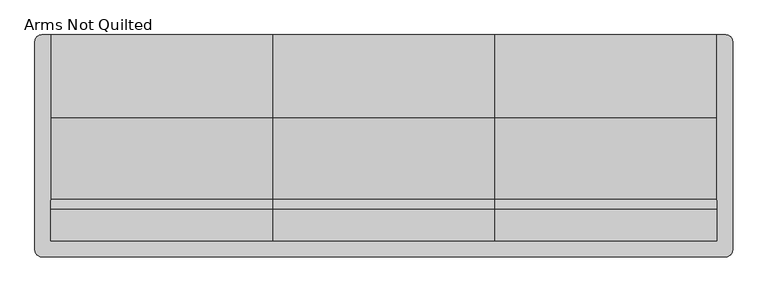
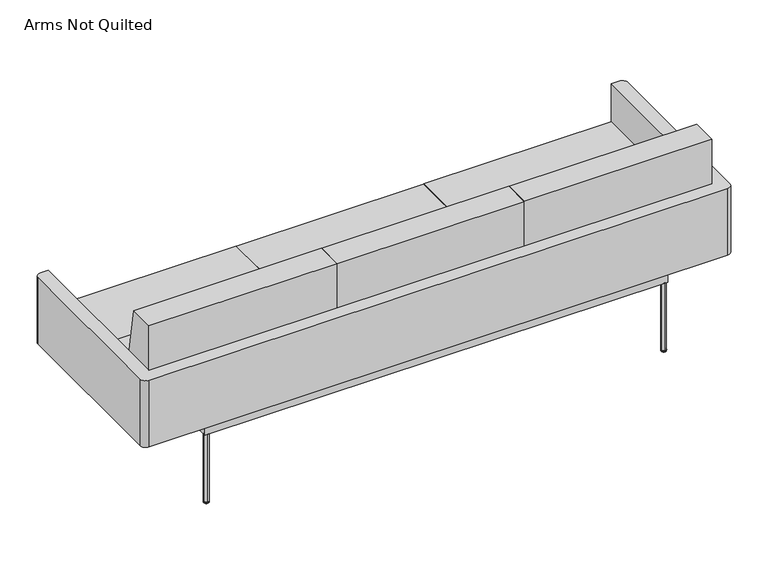
"""IFC4 building model written with IfcOpenShell, lengths in millimetres: furniture geometry, HermanMiller_Collection_Tuxedo_Sofa : Arms Not Quilted."""

from ifc_helpers import new_model, si_unit, point, frame, frame_2d, origin, place, context, project, spatial, polyline, circle_curve, ellipse_curve, trimmed, segment, composite_curve, outline, extrude, source, transform, mapped, element, save
from ifc_brep_helpers import plane_surface, revolved_surface, advanced_brep


def arms_not_quilted_b01c5f5b(model_context):
    return source(origin(), model_context, "Body", "SolidModel", [
        extrude(outline(polyline([(-172.790312, 570.0407405), (-172.790312, 357.1875), (-305.047338, 357.1875), (-305.047338, 761.9999879), (-204.8303749, 761.9999879), (-172.790312, 570.0407405)])), frame((355.8486449, 0.0, 0.0), z_axis=(1.0, 0.0, 0.0), x_axis=(0.0, 1.0, 0.0)), (0.0, 0.0, 1.0), 711.3174324),
        extrude(outline(polyline([(-204.8303749, 761.9999879), (-172.790312, 570.0407405), (-172.790312, 357.1875), (-305.047338, 357.1875), (-305.047338, 761.9999879), (-204.8303749, 761.9999879)])), frame((-1067.1660773, 0.0, 0.0), z_axis=(1.0, 0.0, 0.0), x_axis=(0.0, 1.0, 0.0)), (0.0, 0.0, 1.0), 711.3174324),
        extrude(outline(polyline([(-172.790312, 570.0407405), (-172.790312, 357.1875), (-305.047338, 357.1875), (-305.047338, 761.9999879), (-204.8303749, 761.9999879), (-172.790312, 570.0407405)])), frame((-354.5786449, 0.0, 0.0), z_axis=(1.0, 0.0, 0.0), x_axis=(0.0, 1.0, 0.0)), (0.0, 0.0, 1.0), 709.1572898),
        extrude(outline(polyline([(355.847338, 357.1875), (-172.790312, 357.1875), (-172.790312, 408.4192229), (89.4717005, 431.3641497), (355.847338, 431.3641497), (355.847338, 357.1875)])), frame((355.8486449, 0.0, 0.0), z_axis=(1.0, 0.0, 0.0), x_axis=(0.0, 1.0, 0.0)), (0.0, 0.0, 1.0), 711.3174324),
        extrude(outline(polyline([(355.847338, 431.3641497), (355.847338, 357.1875), (-172.790312, 357.1875), (-172.790312, 408.4192229), (89.4717005, 431.3641497), (355.847338, 431.3641497)])), frame((-1067.1660773, 0.0, 0.0), z_axis=(1.0, 0.0, 0.0), x_axis=(0.0, 1.0, 0.0)), (0.0, 0.0, 1.0), 711.3174324),
        extrude(outline(polyline([(355.847338, 357.1875), (-172.790312, 357.1875), (-172.790312, 408.4192229), (89.4717005, 431.3641497), (355.847338, 431.3641497), (355.847338, 357.1875)])), frame((-354.5786449, 0.0, 0.0), z_axis=(1.0, 0.0, 0.0), x_axis=(0.0, 1.0, 0.0)), (0.0, 0.0, 1.0), 709.1572898),
        advanced_brep(
        [(-862.2241883, 239.6951247, 0.0), (-866.0073712, 239.6951247, 0.0), (-869.7905542, 239.6951247, 0.0), (-856.4823712, 239.6951247, 3.1750001), (-875.5323712, 239.6951247, 3.1750001), (-856.351925, 239.6951247, 6.4931848), (-875.6628174, 239.6951247, 6.4931848), (-861.8574966, 239.6951247, 9.5049435), (-870.1572459, 239.6951247, 9.5049435), (-866.0073712, 239.6951247, 9.5049435)],
        [
            (0, 1),
            (1, 2),
            (2, 0, circle_curve(frame((-866.0073712, 239.6951247, 0.0), z_axis=(0.0, 0.0, -1.0), x_axis=(-1.0, 0.0, 0.0)), 3.783183)),
            (0, 2, circle_curve(frame((-866.0073712, 239.6951247, 0.0), z_axis=(0.0, 0.0, -1.0), x_axis=(-1.0, 0.0, 0.0)), 3.783183)),
            (3, 0, circle_curve(frame((-862.2241883, 239.6951247, 6.7793838), z_axis=(0.0, 1.0, 0.0), x_axis=(1.0, 0.0, 0.0)), 6.7793838)),
            (2, 4, circle_curve(frame((-869.7905542, 239.6951247, 6.7793838), z_axis=(0.0, 1.0, 0.0), x_axis=(-1.0, 0.0, 0.0)), 6.7793838)),
            (4, 3, circle_curve(frame((-866.0073712, 239.6951247, 3.1750001), z_axis=(0.0, 0.0, -1.0), x_axis=(-1.0, 0.0, 0.0)), 9.525)),
            (3, 4, circle_curve(frame((-866.0073712, 239.6951247, 3.1750001), z_axis=(0.0, 0.0, -1.0), x_axis=(-1.0, 0.0, 0.0)), 9.525)),
            (5, 3),
            (4, 6),
            (6, 5, circle_curve(frame((-866.0073712, 239.6951247, 6.4931848), z_axis=(0.0, 0.0, -1.0), x_axis=(-1.0, 0.0, 0.0)), 9.6554462)),
            (5, 6, circle_curve(frame((-866.0073712, 239.6951247, 6.4931848), z_axis=(0.0, 0.0, -1.0), x_axis=(-1.0, 0.0, 0.0)), 9.6554462)),
            (7, 5, circle_curve(frame((-861.8574966, 239.6951247, 2.9669016), z_axis=(0.0, 1.0, 0.0), x_axis=(1.0, 0.0, 0.0)), 6.5380418)),
            (6, 8, circle_curve(frame((-870.1572459, 239.6951247, 2.9669016), z_axis=(0.0, 1.0, 0.0), x_axis=(-1.0, 0.0, 0.0)), 6.5380418)),
            (8, 7, circle_curve(frame((-866.0073712, 239.6951247, 9.5049435), z_axis=(0.0, 0.0, -1.0), x_axis=(-1.0, 0.0, 0.0)), 4.1498747)),
            (7, 8, circle_curve(frame((-866.0073712, 239.6951247, 9.5049435), z_axis=(0.0, 0.0, -1.0), x_axis=(-1.0, 0.0, 0.0)), 4.1498747)),
            (9, 7),
            (8, 9),
        ],
        [
            plane_surface(frame((-866.0073712, 239.6951247, 0.0), z_axis=(0.0, 0.0, -1.0), x_axis=(-1.0, 0.0, 0.0))),
            revolved_surface(trimmed(ellipse_curve(frame((-869.7905542, 239.6951247, 6.7793838), z_axis=(0.0, 1.0, 0.0), x_axis=(-1.0, 0.0, 0.0)), 6.7793838, 6.7793838), [point((-869.7905542, 239.6951247, 0.0))], [point((-875.5323712, 239.6951247, 3.1750001))], True, "CARTESIAN"), (-866.0073712, 239.6951247, 2.4865786), (0.0, 0.0, 1.0)),
            revolved_surface(polyline([(-875.5323712, 239.6951247, 3.1750001), (-875.6628174, 239.6951247, 6.4931848)]), (-866.0073712, 239.6951247, 2.4865786), (0.0, 0.0, 1.0)),
            revolved_surface(trimmed(ellipse_curve(frame((-870.1572459, 239.6951247, 2.9669016), z_axis=(0.0, 1.0, 0.0), x_axis=(-1.0, 0.0, 0.0)), 6.5380418, 6.5380418), [point((-875.6628174, 239.6951247, 6.4931848))], [point((-870.1572459, 239.6951247, 9.5049435))], True, "CARTESIAN"), (-866.0073712, 239.6951247, 2.4865786), (0.0, 0.0, 1.0)),
            plane_surface(frame((-866.0073712, 239.6951247, 9.5049435), z_axis=(0.0, 0.0, 1.0), x_axis=(-1.0, 0.0, 0.0))),
        ],
        [
            (0, [[1, 2, 3]]),
            (0, [[-2, -1, 4]]),
            (1, [[5, -3, 6, 7]]),
            (1, [[-6, -4, -5, 8]]),
            (2, [[9, -7, 10, 11]]),
            (2, [[-10, -8, -9, 12]]),
            (3, [[13, -11, 14, 15]]),
            (3, [[-14, -12, -13, 16]]),
            (4, [[17, -15, 18]]),
            (4, [[-18, -16, -17]]),
        ],
    ),
        advanced_brep(
        [(-866.0073712, -332.5700088, 0.0), (-862.2241883, -332.5700088, 0.0), (-869.7905542, -332.5700088, 0.0), (-856.4823712, -332.5700088, 3.1750001), (-875.5323712, -332.5700088, 3.1750001), (-856.351925, -332.5700088, 6.4931848), (-875.6628174, -332.5700088, 6.4931848), (-861.8574966, -332.5700088, 9.5049435), (-870.1572459, -332.5700088, 9.5049435), (-866.0073712, -332.5700088, 9.5049435)],
        [
            (0, 1),
            (1, 2, circle_curve(frame((-866.0073712, -332.5700088, 0.0), z_axis=(0.0, 0.0, -1.0), x_axis=(-1.0, 0.0, 0.0)), 3.783183)),
            (2, 0),
            (2, 1, circle_curve(frame((-866.0073712, -332.5700088, 0.0), z_axis=(0.0, 0.0, -1.0), x_axis=(-1.0, 0.0, 0.0)), 3.783183)),
            (1, 3, circle_curve(frame((-862.2241883, -332.5700088, 6.7793838), z_axis=(0.0, -1.0, 0.0), x_axis=(1.0, 0.0, 0.0)), 6.7793838)),
            (3, 4, circle_curve(frame((-866.0073712, -332.5700088, 3.1750001), z_axis=(0.0, 0.0, -1.0), x_axis=(-1.0, 0.0, 0.0)), 9.525)),
            (4, 2, circle_curve(frame((-869.7905542, -332.5700088, 6.7793838), z_axis=(0.0, -1.0, 0.0), x_axis=(-1.0, 0.0, 0.0)), 6.7793838)),
            (4, 3, circle_curve(frame((-866.0073712, -332.5700088, 3.1750001), z_axis=(0.0, 0.0, -1.0), x_axis=(-1.0, 0.0, 0.0)), 9.525)),
            (3, 5),
            (5, 6, circle_curve(frame((-866.0073712, -332.5700088, 6.4931848), z_axis=(0.0, 0.0, -1.0), x_axis=(-1.0, 0.0, 0.0)), 9.6554462)),
            (6, 4),
            (6, 5, circle_curve(frame((-866.0073712, -332.5700088, 6.4931848), z_axis=(0.0, 0.0, -1.0), x_axis=(-1.0, 0.0, 0.0)), 9.6554462)),
            (5, 7, circle_curve(frame((-861.8574966, -332.5700088, 2.9669016), z_axis=(0.0, -1.0, 0.0), x_axis=(1.0, 0.0, 0.0)), 6.5380418)),
            (7, 8, circle_curve(frame((-866.0073712, -332.5700088, 9.5049435), z_axis=(0.0, 0.0, -1.0), x_axis=(-1.0, 0.0, 0.0)), 4.1498747)),
            (8, 6, circle_curve(frame((-870.1572459, -332.5700088, 2.9669016), z_axis=(0.0, -1.0, 0.0), x_axis=(-1.0, 0.0, 0.0)), 6.5380418)),
            (8, 7, circle_curve(frame((-866.0073712, -332.5700088, 9.5049435), z_axis=(0.0, 0.0, -1.0), x_axis=(-1.0, 0.0, 0.0)), 4.1498747)),
            (7, 9),
            (9, 8),
        ],
        [
            plane_surface(frame((-866.0073712, -332.5700088, 0.0), z_axis=(0.0, 0.0, -1.0), x_axis=(-1.0, 0.0, 0.0))),
            revolved_surface(trimmed(ellipse_curve(frame((-869.7905542, -332.5700088, 6.7793838), z_axis=(0.0, -1.0, 0.0), x_axis=(-1.0, 0.0, 0.0)), 6.7793838, 6.7793838), [point((-875.5323712, -332.5700088, 3.1750001))], [point((-869.7905542, -332.5700088, 0.0))], True, "CARTESIAN"), (-866.0073712, -332.5700088, 2.4865786), (0.0, 0.0, -1.0)),
            revolved_surface(polyline([(-875.6628174, -332.5700088, 6.4931848), (-875.5323712, -332.5700088, 3.1750001)]), (-866.0073712, -332.5700088, 2.4865786), (0.0, 0.0, -1.0)),
            revolved_surface(trimmed(ellipse_curve(frame((-870.1572459, -332.5700088, 2.9669016), z_axis=(0.0, -1.0, 0.0), x_axis=(-1.0, 0.0, 0.0)), 6.5380418, 6.5380418), [point((-870.1572459, -332.5700088, 9.5049435))], [point((-875.6628174, -332.5700088, 6.4931848))], True, "CARTESIAN"), (-866.0073712, -332.5700088, 2.4865786), (0.0, 0.0, -1.0)),
            plane_surface(frame((-866.0073712, -332.5700088, 9.5049435), z_axis=(0.0, 0.0, 1.0), x_axis=(-1.0, 0.0, 0.0))),
        ],
        [
            (0, [[1, 2, 3]]),
            (0, [[-3, 4, -1]]),
            (1, [[5, 6, 7, -2]]),
            (1, [[-7, 8, -5, -4]]),
            (2, [[9, 10, 11, -6]]),
            (2, [[-11, 12, -9, -8]]),
            (3, [[13, 14, 15, -10]]),
            (3, [[-15, 16, -13, -12]]),
            (4, [[17, 18, -14]]),
            (4, [[-18, -17, -16]]),
        ],
    ),
        extrude(outline(composite_curve([segment(polyline([(-1117.9660773, -333.876338), (-1117.9660773, 333.876338)]), True, "CONTINUOUS"), segment(trimmed(circle_curve(frame_2d((-1095.9950773, 333.876338)), 21.971), [point((-1117.9660773, 333.876338))], [point((-1095.9950773, 355.847338))], False, "CARTESIAN"), True, "CONTINUOUS"), segment(polyline([(-1095.9950773, 355.847338), (-1067.1660773, 355.847338), (-1067.1660773, -305.047338), (1067.1660773, -305.047338), (1067.1660773, 355.847338), (1095.9994733, 355.847338)]), True, "CONTINUOUS"), segment(trimmed(circle_curve(frame_2d((1095.9994733, 333.880734)), 21.966604), [point((1095.9994733, 355.847338))], [point((1117.9660773, 333.880734))], False, "CARTESIAN"), True, "CONTINUOUS"), segment(polyline([(1117.9660773, 333.880734), (1117.9660773, -333.876338)]), True, "CONTINUOUS"), segment(trimmed(circle_curve(frame_2d((1095.9950773, -333.876338)), 21.971), [point((1117.9660773, -333.876338))], [point((1095.9950773, -355.847338))], False, "CARTESIAN"), True, "CONTINUOUS"), segment(polyline([(1095.9950773, -355.847338), (-1095.9950773, -355.847338)]), True, "CONTINUOUS"), segment(trimmed(circle_curve(frame_2d((-1095.9950773, -333.876338)), 21.971), [point((-1095.9950773, -355.847338))], [point((-1117.9660773, -333.876338))], False, "CARTESIAN"), True, "CONTINUOUS")], self_intersect=False)), frame((0.0, 0.0, 317.4993339), z_axis=(0.0, 0.0, 1.0), x_axis=(1.0, 0.0, 0.0)), (0.0, 0.0, 1.0), 266.700654),
        extrude(outline(composite_curve([segment(trimmed(circle_curve(frame_2d((-865.5330732, -332.8903279)), 9.525), [point((-875.0580732, -332.8903279))], [point((-865.5330732, -323.3653279))], False, "CARTESIAN"), True, "CONTINUOUS"), segment(trimmed(circle_curve(frame_2d((-865.5330732, -332.8903279)), 9.525), [point((-865.5330732, -323.3653279))], [point((-856.0080732, -332.8903279))], False, "CARTESIAN"), True, "CONTINUOUS"), segment(trimmed(circle_curve(frame_2d((-865.5330732, -332.8903279)), 9.525), [point((-856.0080732, -332.8903279))], [point((-865.5330732, -342.4153279))], False, "CARTESIAN"), True, "CONTINUOUS"), segment(trimmed(circle_curve(frame_2d((-865.5330732, -332.8903279)), 9.525), [point((-865.5330732, -342.4153279))], [point((-875.0580732, -332.8903279))], False, "CARTESIAN"), True, "CONTINUOUS")], self_intersect=False)), frame((0.0, 0.0, 9.525), z_axis=(0.0, 0.0, 1.0), x_axis=(1.0, 0.0, 0.0)), (0.0, 0.0, 1.0), 269.8750061),
        extrude(outline(composite_curve([segment(trimmed(circle_curve(frame_2d((-865.4343312, 238.7745677)), 9.525), [point((-874.9593312, 238.7745677))], [point((-865.4343312, 248.2995677))], False, "CARTESIAN"), True, "CONTINUOUS"), segment(trimmed(circle_curve(frame_2d((-865.4343312, 238.7745677)), 9.525), [point((-865.4343312, 248.2995677))], [point((-855.9093312, 238.7745677))], False, "CARTESIAN"), True, "CONTINUOUS"), segment(trimmed(circle_curve(frame_2d((-865.4343312, 238.7745677)), 9.525), [point((-855.9093312, 238.7745677))], [point((-865.4343312, 229.2495677))], False, "CARTESIAN"), True, "CONTINUOUS"), segment(trimmed(circle_curve(frame_2d((-865.4343312, 238.7745677)), 9.525), [point((-865.4343312, 229.2495677))], [point((-874.9593312, 238.7745677))], False, "CARTESIAN"), True, "CONTINUOUS")], self_intersect=False)), frame((0.0, 0.0, 9.525), z_axis=(0.0, 0.0, 1.0), x_axis=(1.0, 0.0, 0.0)), (0.0, 0.0, 1.0), 269.8750061),
        advanced_brep(
        [(-861.749631, 238.459695, 0.0), (-865.532814, 238.459695, 0.0), (-869.3159969, 238.459695, 0.0), (-856.007814, 238.459695, 3.1750001), (-875.057814, 238.459695, 3.1750001), (-855.8773678, 238.459695, 6.4931848), (-875.1882602, 238.459695, 6.4931848), (-861.3829393, 238.459695, 9.5049435), (-869.6826886, 238.459695, 9.5049435), (-865.532814, 238.459695, 9.5049435)],
        [
            (0, 1),
            (1, 2),
            (2, 0, circle_curve(frame((-865.532814, 238.459695, 0.0), z_axis=(0.0, 0.0, -1.0), x_axis=(-1.0, 0.0, 0.0)), 3.783183)),
            (0, 2, circle_curve(frame((-865.532814, 238.459695, 0.0), z_axis=(0.0, 0.0, -1.0), x_axis=(-1.0, 0.0, 0.0)), 3.783183)),
            (3, 0, circle_curve(frame((-861.749631, 238.459695, 6.7793838), z_axis=(0.0, 1.0, 0.0), x_axis=(1.0, 0.0, 0.0)), 6.7793838)),
            (2, 4, circle_curve(frame((-869.3159969, 238.459695, 6.7793838), z_axis=(0.0, 1.0, 0.0), x_axis=(-1.0, 0.0, 0.0)), 6.7793838)),
            (4, 3, circle_curve(frame((-865.532814, 238.459695, 3.1750001), z_axis=(0.0, 0.0, -1.0), x_axis=(-1.0, 0.0, 0.0)), 9.525)),
            (3, 4, circle_curve(frame((-865.532814, 238.459695, 3.1750001), z_axis=(0.0, 0.0, -1.0), x_axis=(-1.0, 0.0, 0.0)), 9.525)),
            (5, 3),
            (4, 6),
            (6, 5, circle_curve(frame((-865.532814, 238.459695, 6.4931848), z_axis=(0.0, 0.0, -1.0), x_axis=(-1.0, 0.0, 0.0)), 9.6554462)),
            (5, 6, circle_curve(frame((-865.532814, 238.459695, 6.4931848), z_axis=(0.0, 0.0, -1.0), x_axis=(-1.0, 0.0, 0.0)), 9.6554462)),
            (7, 5, circle_curve(frame((-861.3829393, 238.459695, 2.9669016), z_axis=(0.0, 1.0, 0.0), x_axis=(1.0, 0.0, 0.0)), 6.5380418)),
            (6, 8, circle_curve(frame((-869.6826886, 238.459695, 2.9669016), z_axis=(0.0, 1.0, 0.0), x_axis=(-1.0, 0.0, 0.0)), 6.5380418)),
            (8, 7, circle_curve(frame((-865.532814, 238.459695, 9.5049435), z_axis=(0.0, 0.0, -1.0), x_axis=(-1.0, 0.0, 0.0)), 4.1498747)),
            (7, 8, circle_curve(frame((-865.532814, 238.459695, 9.5049435), z_axis=(0.0, 0.0, -1.0), x_axis=(-1.0, 0.0, 0.0)), 4.1498747)),
            (9, 7),
            (8, 9),
        ],
        [
            plane_surface(frame((-865.532814, 238.459695, 0.0), z_axis=(0.0, 0.0, -1.0), x_axis=(-1.0, 0.0, 0.0))),
            revolved_surface(trimmed(ellipse_curve(frame((-869.3159969, 238.459695, 6.7793838), z_axis=(0.0, 1.0, 0.0), x_axis=(-1.0, 0.0, 0.0)), 6.7793838, 6.7793838), [point((-869.3159969, 238.459695, 0.0))], [point((-875.057814, 238.459695, 3.1750001))], True, "CARTESIAN"), (-865.532814, 238.459695, 2.4865786), (0.0, 0.0, 1.0)),
            revolved_surface(polyline([(-875.057814, 238.459695, 3.1750001), (-875.1882602, 238.459695, 6.4931848)]), (-865.532814, 238.459695, 2.4865786), (0.0, 0.0, 1.0)),
            revolved_surface(trimmed(ellipse_curve(frame((-869.6826886, 238.459695, 2.9669016), z_axis=(0.0, 1.0, 0.0), x_axis=(-1.0, 0.0, 0.0)), 6.5380418, 6.5380418), [point((-875.1882602, 238.459695, 6.4931848))], [point((-869.6826886, 238.459695, 9.5049435))], True, "CARTESIAN"), (-865.532814, 238.459695, 2.4865786), (0.0, 0.0, 1.0)),
            plane_surface(frame((-865.532814, 238.459695, 9.5049435), z_axis=(0.0, 0.0, 1.0), x_axis=(-1.0, 0.0, 0.0))),
        ],
        [
            (0, [[1, 2, 3]]),
            (0, [[-2, -1, 4]]),
            (1, [[5, -3, 6, 7]]),
            (1, [[-6, -4, -5, 8]]),
            (2, [[9, -7, 10, 11]]),
            (2, [[-10, -8, -9, 12]]),
            (3, [[13, -11, 14, 15]]),
            (3, [[-14, -12, -13, 16]]),
            (4, [[17, -15, 18]]),
            (4, [[-18, -16, -17]]),
        ],
    ),
        advanced_brep(
        [(-865.8408432, -332.7425888, 0.0), (-862.0576602, -332.7425888, 0.0), (-869.6240261, -332.7425888, 0.0), (-856.3158432, -332.7425888, 3.1750001), (-875.3658432, -332.7425888, 3.1750001), (-856.185397, -332.7425888, 6.4931848), (-875.4962893, -332.7425888, 6.4931848), (-861.6909685, -332.7425888, 9.5049435), (-869.9907178, -332.7425888, 9.5049435), (-865.8408432, -332.7425888, 9.5049435)],
        [
            (0, 1),
            (1, 2, circle_curve(frame((-865.8408432, -332.7425888, 0.0), z_axis=(0.0, 0.0, -1.0), x_axis=(-1.0, 0.0, 0.0)), 3.783183)),
            (2, 0),
            (2, 1, circle_curve(frame((-865.8408432, -332.7425888, 0.0), z_axis=(0.0, 0.0, -1.0), x_axis=(-1.0, 0.0, 0.0)), 3.783183)),
            (1, 3, circle_curve(frame((-862.0576602, -332.7425888, 6.7793838), z_axis=(0.0, -1.0, 0.0), x_axis=(1.0, 0.0, 0.0)), 6.7793838)),
            (3, 4, circle_curve(frame((-865.8408432, -332.7425888, 3.1750001), z_axis=(0.0, 0.0, -1.0), x_axis=(-1.0, 0.0, 0.0)), 9.525)),
            (4, 2, circle_curve(frame((-869.6240261, -332.7425888, 6.7793838), z_axis=(0.0, -1.0, 0.0), x_axis=(-1.0, 0.0, 0.0)), 6.7793838)),
            (4, 3, circle_curve(frame((-865.8408432, -332.7425888, 3.1750001), z_axis=(0.0, 0.0, -1.0), x_axis=(-1.0, 0.0, 0.0)), 9.525)),
            (3, 5),
            (5, 6, circle_curve(frame((-865.8408432, -332.7425888, 6.4931848), z_axis=(0.0, 0.0, -1.0), x_axis=(-1.0, 0.0, 0.0)), 9.6554462)),
            (6, 4),
            (6, 5, circle_curve(frame((-865.8408432, -332.7425888, 6.4931848), z_axis=(0.0, 0.0, -1.0), x_axis=(-1.0, 0.0, 0.0)), 9.6554462)),
            (5, 7, circle_curve(frame((-861.6909685, -332.7425888, 2.9669016), z_axis=(0.0, -1.0, 0.0), x_axis=(1.0, 0.0, 0.0)), 6.5380418)),
            (7, 8, circle_curve(frame((-865.8408432, -332.7425888, 9.5049435), z_axis=(0.0, 0.0, -1.0), x_axis=(-1.0, 0.0, 0.0)), 4.1498747)),
            (8, 6, circle_curve(frame((-869.9907178, -332.7425888, 2.9669016), z_axis=(0.0, -1.0, 0.0), x_axis=(-1.0, 0.0, 0.0)), 6.5380418)),
            (8, 7, circle_curve(frame((-865.8408432, -332.7425888, 9.5049435), z_axis=(0.0, 0.0, -1.0), x_axis=(-1.0, 0.0, 0.0)), 4.1498747)),
            (7, 9),
            (9, 8),
        ],
        [
            plane_surface(frame((-865.8408432, -332.7425888, 0.0), z_axis=(0.0, 0.0, -1.0), x_axis=(-1.0, 0.0, 0.0))),
            revolved_surface(trimmed(ellipse_curve(frame((-869.6240261, -332.7425888, 6.7793838), z_axis=(0.0, -1.0, 0.0), x_axis=(-1.0, 0.0, 0.0)), 6.7793838, 6.7793838), [point((-875.3658432, -332.7425888, 3.1750001))], [point((-869.6240261, -332.7425888, 0.0))], True, "CARTESIAN"), (-865.8408432, -332.7425888, 2.4865786), (0.0, 0.0, -1.0)),
            revolved_surface(polyline([(-875.4962893, -332.7425888, 6.4931848), (-875.3658432, -332.7425888, 3.1750001)]), (-865.8408432, -332.7425888, 2.4865786), (0.0, 0.0, -1.0)),
            revolved_surface(trimmed(ellipse_curve(frame((-869.9907178, -332.7425888, 2.9669016), z_axis=(0.0, -1.0, 0.0), x_axis=(-1.0, 0.0, 0.0)), 6.5380418, 6.5380418), [point((-869.9907178, -332.7425888, 9.5049435))], [point((-875.4962893, -332.7425888, 6.4931848))], True, "CARTESIAN"), (-865.8408432, -332.7425888, 2.4865786), (0.0, 0.0, -1.0)),
            plane_surface(frame((-865.8408432, -332.7425888, 9.5049435), z_axis=(0.0, 0.0, 1.0), x_axis=(-1.0, 0.0, 0.0))),
        ],
        [
            (0, [[1, 2, 3]]),
            (0, [[-3, 4, -1]]),
            (1, [[5, 6, 7, -2]]),
            (1, [[-7, 8, -5, -4]]),
            (2, [[9, 10, 11, -6]]),
            (2, [[-11, 12, -9, -8]]),
            (3, [[13, 14, 15, -10]]),
            (3, [[-15, 16, -13, -12]]),
            (4, [[17, 18, -14]]),
            (4, [[-18, -17, -16]]),
        ],
    ),
        advanced_brep(
        [(867.9917462, 239.6951247, 0.0), (864.2085633, 239.6951247, 0.0), (871.7749292, 239.6951247, 0.0), (858.4667462, 239.6951247, 3.1750001), (877.5167462, 239.6951247, 3.1750001), (858.3363, 239.6951247, 6.4931848), (877.6471924, 239.6951247, 6.4931848), (863.8418716, 239.6951247, 9.5049434), (872.1416209, 239.6951247, 9.5049434), (867.9917462, 239.6951247, 9.5049435)],
        [
            (0, 1),
            (1, 2, circle_curve(frame((867.9917462, 239.6951247, 0.0), z_axis=(0.0, 0.0, -1.0), x_axis=(1.0, 0.0, 0.0)), 3.783183)),
            (2, 0),
            (2, 1, circle_curve(frame((867.9917462, 239.6951247, 0.0), z_axis=(0.0, 0.0, -1.0), x_axis=(1.0, 0.0, 0.0)), 3.783183)),
            (1, 3, circle_curve(frame((864.2085633, 239.6951247, 6.7793838), z_axis=(0.0, 1.0, 0.0), x_axis=(-1.0, 0.0, 0.0)), 6.7793838)),
            (3, 4, circle_curve(frame((867.9917462, 239.6951247, 3.1750001), z_axis=(0.0, 0.0, -1.0), x_axis=(1.0, 0.0, 0.0)), 9.525)),
            (4, 2, circle_curve(frame((871.7749292, 239.6951247, 6.7793838), z_axis=(0.0, 1.0, 0.0), x_axis=(1.0, 0.0, 0.0)), 6.7793838)),
            (4, 3, circle_curve(frame((867.9917462, 239.6951247, 3.1750001), z_axis=(0.0, 0.0, -1.0), x_axis=(1.0, 0.0, 0.0)), 9.525)),
            (3, 5),
            (5, 6, circle_curve(frame((867.9917462, 239.6951247, 6.4931848), z_axis=(0.0, 0.0, -1.0), x_axis=(1.0, 0.0, 0.0)), 9.6554462)),
            (6, 4),
            (6, 5, circle_curve(frame((867.9917462, 239.6951247, 6.4931848), z_axis=(0.0, 0.0, -1.0), x_axis=(1.0, 0.0, 0.0)), 9.6554462)),
            (5, 7, circle_curve(frame((863.8418716, 239.6951247, 2.9669016), z_axis=(0.0, 1.0, 0.0), x_axis=(-1.0, 0.0, 0.0)), 6.5380418)),
            (7, 8, circle_curve(frame((867.9917462, 239.6951247, 9.5049434), z_axis=(0.0, 0.0, -1.0), x_axis=(1.0, 0.0, 0.0)), 4.1498747)),
            (8, 6, circle_curve(frame((872.1416209, 239.6951247, 2.9669016), z_axis=(0.0, 1.0, 0.0), x_axis=(1.0, 0.0, 0.0)), 6.5380418)),
            (8, 7, circle_curve(frame((867.9917462, 239.6951247, 9.5049434), z_axis=(0.0, 0.0, -1.0), x_axis=(1.0, 0.0, 0.0)), 4.1498747)),
            (7, 9),
            (9, 8),
        ],
        [
            plane_surface(frame((867.9917462, 239.6951247, 0.0), z_axis=(0.0, 0.0, -1.0), x_axis=(1.0, 0.0, 0.0))),
            revolved_surface(trimmed(ellipse_curve(frame((871.7749292, 239.6951247, 6.7793838), z_axis=(0.0, 1.0, 0.0), x_axis=(1.0, 0.0, 0.0)), 6.7793838, 6.7793838), [point((877.5167462, 239.6951247, 3.1750001))], [point((871.7749292, 239.6951247, 0.0))], True, "CARTESIAN"), (867.9917462, 239.6951247, 2.4865786), (0.0, 0.0, -1.0)),
            revolved_surface(polyline([(877.6471924, 239.6951247, 6.4931848), (877.5167462, 239.6951247, 3.1750001)]), (867.9917462, 239.6951247, 2.4865786), (0.0, 0.0, -1.0)),
            revolved_surface(trimmed(ellipse_curve(frame((872.1416209, 239.6951247, 2.9669016), z_axis=(0.0, 1.0, 0.0), x_axis=(1.0, 0.0, 0.0)), 6.5380418, 6.5380418), [point((872.1416209, 239.6951247, 9.5049434))], [point((877.6471924, 239.6951247, 6.4931848))], True, "CARTESIAN"), (867.9917462, 239.6951247, 2.4865786), (0.0, 0.0, -1.0)),
            plane_surface(frame((867.9917462, 239.6951247, 9.5049435), z_axis=(0.0, 0.0, 1.0), x_axis=(1.0, 0.0, 0.0))),
        ],
        [
            (0, [[1, 2, 3]]),
            (0, [[-3, 4, -1]]),
            (1, [[5, 6, 7, -2]]),
            (1, [[-7, 8, -5, -4]]),
            (2, [[9, 10, 11, -6]]),
            (2, [[-11, 12, -9, -8]]),
            (3, [[13, 14, 15, -10]]),
            (3, [[-15, 16, -13, -12]]),
            (4, [[17, 18, -14]]),
            (4, [[-18, -17, -16]]),
        ],
    ),
        advanced_brep(
        [(864.2085633, -332.5700088, 0.0), (867.9917462, -332.5700088, 0.0), (871.7749292, -332.5700088, 0.0), (858.4667462, -332.5700088, 3.1750001), (877.5167462, -332.5700088, 3.1750001), (858.3363, -332.5700088, 6.4931848), (877.6471924, -332.5700088, 6.4931848), (863.8418716, -332.5700088, 9.5049435), (872.1416209, -332.5700088, 9.5049435), (867.9917462, -332.5700088, 9.5049435)],
        [
            (0, 1),
            (1, 2),
            (2, 0, circle_curve(frame((867.9917462, -332.5700088, 0.0), z_axis=(0.0, 0.0, -1.0), x_axis=(1.0, 0.0, 0.0)), 3.783183)),
            (0, 2, circle_curve(frame((867.9917462, -332.5700088, 0.0), z_axis=(0.0, 0.0, -1.0), x_axis=(1.0, 0.0, 0.0)), 3.783183)),
            (3, 0, circle_curve(frame((864.2085633, -332.5700088, 6.7793838), z_axis=(0.0, -1.0, 0.0), x_axis=(-1.0, 0.0, 0.0)), 6.7793838)),
            (2, 4, circle_curve(frame((871.7749292, -332.5700088, 6.7793838), z_axis=(0.0, -1.0, 0.0), x_axis=(1.0, 0.0, 0.0)), 6.7793838)),
            (4, 3, circle_curve(frame((867.9917462, -332.5700088, 3.1750001), z_axis=(0.0, 0.0, -1.0), x_axis=(1.0, 0.0, 0.0)), 9.525)),
            (3, 4, circle_curve(frame((867.9917462, -332.5700088, 3.1750001), z_axis=(0.0, 0.0, -1.0), x_axis=(1.0, 0.0, 0.0)), 9.525)),
            (5, 3),
            (4, 6),
            (6, 5, circle_curve(frame((867.9917462, -332.5700088, 6.4931848), z_axis=(0.0, 0.0, -1.0), x_axis=(1.0, 0.0, 0.0)), 9.6554462)),
            (5, 6, circle_curve(frame((867.9917462, -332.5700088, 6.4931848), z_axis=(0.0, 0.0, -1.0), x_axis=(1.0, 0.0, 0.0)), 9.6554462)),
            (7, 5, circle_curve(frame((863.8418716, -332.5700088, 2.9669016), z_axis=(0.0, -1.0, 0.0), x_axis=(-1.0, 0.0, 0.0)), 6.5380418)),
            (6, 8, circle_curve(frame((872.1416209, -332.5700088, 2.9669016), z_axis=(0.0, -1.0, 0.0), x_axis=(1.0, 0.0, 0.0)), 6.5380418)),
            (8, 7, circle_curve(frame((867.9917462, -332.5700088, 9.5049435), z_axis=(0.0, 0.0, -1.0), x_axis=(1.0, 0.0, 0.0)), 4.1498747)),
            (7, 8, circle_curve(frame((867.9917462, -332.5700088, 9.5049435), z_axis=(0.0, 0.0, -1.0), x_axis=(1.0, 0.0, 0.0)), 4.1498747)),
            (9, 7),
            (8, 9),
        ],
        [
            plane_surface(frame((867.9917462, -332.5700088, 0.0), z_axis=(0.0, 0.0, -1.0), x_axis=(1.0, 0.0, 0.0))),
            revolved_surface(trimmed(ellipse_curve(frame((871.7749292, -332.5700088, 6.7793838), z_axis=(0.0, -1.0, 0.0), x_axis=(1.0, 0.0, 0.0)), 6.7793838, 6.7793838), [point((871.7749292, -332.5700088, 0.0))], [point((877.5167462, -332.5700088, 3.1750001))], True, "CARTESIAN"), (867.9917462, -332.5700088, 2.4865786), (0.0, 0.0, 1.0)),
            revolved_surface(polyline([(877.5167462, -332.5700088, 3.1750001), (877.6471924, -332.5700088, 6.4931848)]), (867.9917462, -332.5700088, 2.4865786), (0.0, 0.0, 1.0)),
            revolved_surface(trimmed(ellipse_curve(frame((872.1416209, -332.5700088, 2.9669016), z_axis=(0.0, -1.0, 0.0), x_axis=(1.0, 0.0, 0.0)), 6.5380418, 6.5380418), [point((877.6471924, -332.5700088, 6.4931848))], [point((872.1416209, -332.5700088, 9.5049435))], True, "CARTESIAN"), (867.9917462, -332.5700088, 2.4865786), (0.0, 0.0, 1.0)),
            plane_surface(frame((867.9917462, -332.5700088, 9.5049435), z_axis=(0.0, 0.0, 1.0), x_axis=(1.0, 0.0, 0.0))),
        ],
        [
            (0, [[1, 2, 3]]),
            (0, [[-2, -1, 4]]),
            (1, [[5, -3, 6, 7]]),
            (1, [[-6, -4, -5, 8]]),
            (2, [[9, -7, 10, 11]]),
            (2, [[-10, -8, -9, 12]]),
            (3, [[13, -11, 14, 15]]),
            (3, [[-14, -12, -13, 16]]),
            (4, [[17, -15, 18]]),
            (4, [[-18, -16, -17]]),
        ],
    ),
        extrude(outline(composite_curve([segment(trimmed(circle_curve(frame_2d((867.5174482, -332.8903279)), 9.525), [point((877.0424482, -332.8903279))], [point((867.5174482, -342.4153279))], False, "CARTESIAN"), True, "CONTINUOUS"), segment(trimmed(circle_curve(frame_2d((867.5174482, -332.8903279)), 9.525), [point((867.5174482, -342.4153279))], [point((857.9924482, -332.8903279))], False, "CARTESIAN"), True, "CONTINUOUS"), segment(trimmed(circle_curve(frame_2d((867.5174482, -332.8903279)), 9.525), [point((857.9924482, -332.8903279))], [point((867.5174482, -323.3653279))], False, "CARTESIAN"), True, "CONTINUOUS"), segment(trimmed(circle_curve(frame_2d((867.5174482, -332.8903279)), 9.525), [point((867.5174482, -323.3653279))], [point((877.0424482, -332.8903279))], False, "CARTESIAN"), True, "CONTINUOUS")], self_intersect=False)), frame((0.0, 0.0, 9.525), z_axis=(0.0, 0.0, 1.0), x_axis=(1.0, 0.0, 0.0)), (0.0, 0.0, 1.0), 269.8750061),
        extrude(outline(composite_curve([segment(trimmed(circle_curve(frame_2d((867.4187062, 238.7745677)), 9.525), [point((876.9437062, 238.7745677))], [point((867.4187062, 229.2495677))], False, "CARTESIAN"), True, "CONTINUOUS"), segment(trimmed(circle_curve(frame_2d((867.4187062, 238.7745677)), 9.525), [point((867.4187062, 229.2495677))], [point((857.8937062, 238.7745677))], False, "CARTESIAN"), True, "CONTINUOUS"), segment(trimmed(circle_curve(frame_2d((867.4187062, 238.7745677)), 9.525), [point((857.8937062, 238.7745677))], [point((867.4187062, 248.2995677))], False, "CARTESIAN"), True, "CONTINUOUS"), segment(trimmed(circle_curve(frame_2d((867.4187062, 238.7745677)), 9.525), [point((867.4187062, 248.2995677))], [point((876.9437062, 238.7745677))], False, "CARTESIAN"), True, "CONTINUOUS")], self_intersect=False)), frame((0.0, 0.0, 9.525), z_axis=(0.0, 0.0, 1.0), x_axis=(1.0, 0.0, 0.0)), (0.0, 0.0, 1.0), 269.8750061),
        extrude(outline(polyline([(877.2925536, -342.5689221), (-877.2925536, -342.5689221), (-877.2925536, 248.3227239), (877.2925536, 248.3227239), (877.2925536, -342.5689221)]), holes=[polyline([(858.2425536, -323.5189221), (858.2425536, 229.2727239), (-858.2425536, 229.2727239), (-858.2425536, -323.5189221), (858.2425536, -323.5189221)])]), frame((0.0, 0.0, 279.4000061), z_axis=(0.0, 0.0, 1.0), x_axis=(1.0, 0.0, 0.0)), (0.0, 0.0, 1.0), 38.0999818),
        extrude(outline(polyline([(-1067.1660773, -305.047338), (-1067.1660773, 355.847338), (1067.1660773, 355.847338), (1067.1660773, -305.047338), (-1067.1660773, -305.047338)])), frame((0.0, 0.0, 318.7699879), z_axis=(0.0, 0.0, 1.0), x_axis=(1.0, 0.0, 0.0)), (0.0, 0.0, 1.0), 37.1475121),
    ])


if __name__ == "__main__":
    model = new_model("IFC4")
    model_context = context("Model", 3, world=origin())
    ifc_project = project(units=[si_unit("LENGTHUNIT", "METRE", prefix="MILLI")], contexts=[model_context])
    site = spatial("IfcSite", under=ifc_project)
    building = spatial("IfcBuilding", under=site)
    placement = place(None, origin())
    arms_not_quilted_shape = arms_not_quilted_b01c5f5b(model_context)
    element("IfcFurniture", 1, ObjectType="HermanMiller_Collection_Tuxedo_Sofa : Arms Not Quilted", at=placement, inside=building, context=model_context, shape_type="MappedRepresentation", body=[
        mapped(arms_not_quilted_shape, transform((0.0, 0.0, 0.0), x_axis=(1.0, 0.0, 0.0), y_axis=(0.0, 1.0, 0.0), z_axis=(0.0, 0.0, 1.0))),
    ])
    save(model, "model.ifc")

# Revit data of these elements
# Type "HermanMiller_Collection_Tuxedo_Sofa : Arms Not Quilted"
#   Watermarked By = "http://revitwatermark.com"
#   URL = "http://www.hermanmiller.com\r\n"
#   Product Documentation Link = "http://www.hermanmiller.com/products/seating/lounge-seating/tuxedo-lounge-seating.html"
#   Model = "ST3AN"
#   Manufacturer = "Herman Miller, Inc."
#   Description = "Tuxedo Sofa Arms Not Quilted"
#   Copyright © = "Copyright © Herman Miller, Inc."
#   Catalog Code = "HMH"
#   Catalog = "Herman Miller Collection"
#   Base Price [instance default] = ""
#   Assembly Code = "E2020200"
#   spacing = 0' - 2.91982"
#   quiltLength = 0' - 6.85"
#   quiltHeight = 0' - 3.3"
#   quiltGapHalf = 0' - 0.075"
#   quiltGap = 0' - 0.15"
#   quiltEdgeGap = 0' - 0.83941"
#   quilt Length = 0' - 7"
#   quilt Height = 0' - 3.35"
#   frameThickness = 0' - 0 3/4"
#   cutHeight [instance default] = 0' - 4.4"
#   Arm Thicknes = 0' - 2"
#   Quilted [instance default] = no
#   Package Qty = 1
#   Not Quilted [instance default] = yes
#   Has Arms [instance default] = yes
#   Arms Off [instance default] = no
#   Upholstery [instance default] = Herman Miller - Seat Fabric 8R18 Twist Sepia
#   Base Finish [instance default] = Herman Miller - Finish AS Arctic Silver
#   Type Comments = ""
# Element 1 (IfcFurniture, "HermanMiller_Collection_Tuxedo_Sofa : Arms Not Quilted")
#   Materials on its faces: "Herman Miller - Finish AS Arctic Silver", "Herman Miller - Seat Fabric 8R18 Twist Sepia"
# Materials
#   "Herman Miller - Seat Fabric 8R18 Twist Sepia": class "Unassigned", colour RGB 132 112 87, transparency 0, Keynote = "﻿﻿         ﻿                      ​     ​   ​  ﻿   ​                   ﻿       ﻿   ﻿           ​  ​   ​                ﻿        ﻿  ﻿      ﻿  ﻿      ​     ﻿                       ﻿ ​ ​   ﻿    ​​       ﻿            ﻿﻿﻿﻿               ﻿      ﻿   ﻿﻿​ ﻿         ﻿    ﻿        ​      ​   ﻿  ​ ﻿         ﻿ ​     ﻿                ﻿﻿", Comments = "﻿﻿         ﻿                      ​     ​   ​  ﻿   ​                   ﻿       ﻿   ﻿           ​  ​   ​                ﻿        ﻿  ﻿      ﻿  ﻿      ​     ﻿                       ﻿ ​ ​   ﻿    ​​       ﻿            ﻿﻿﻿﻿               ﻿      ﻿   ﻿﻿​ ﻿         ﻿    ﻿        ​      ​   ﻿  ​ ﻿         ﻿ ​     ﻿                ﻿﻿", Description = "﻿﻿         ﻿                      ​     ​   ​  ﻿   ​                   ﻿       ﻿   ﻿           ​  ​   ​                ﻿        ﻿  ﻿      ﻿  ﻿      ​     ﻿                       ﻿ ​ ​   ﻿    ​​       ﻿            ﻿﻿﻿﻿               ﻿      ﻿   ﻿﻿​ ﻿         ﻿    ﻿        ​      ​   ﻿  ​ ﻿         ﻿ ​     ﻿                ﻿﻿"
#   "Herman Miller - Finish AS Arctic Silver": class "Plastic", colour RGB 188 188 191, transparency 0, Keynote = "﻿﻿         ﻿                      ​     ​   ​  ﻿   ​                   ﻿       ﻿   ﻿           ​  ​   ​                ﻿        ﻿  ﻿      ﻿  ﻿      ​     ﻿                       ﻿ ​ ​   ﻿    ​​       ﻿            ﻿﻿﻿﻿               ﻿      ﻿   ﻿﻿​ ﻿         ﻿    ﻿        ​      ​   ﻿  ​ ﻿         ﻿ ​     ﻿                ﻿﻿", Comments = "﻿﻿         ﻿                      ​     ​   ​  ﻿   ​                   ﻿       ﻿   ﻿           ​  ​   ​                ﻿        ﻿  ﻿      ﻿  ﻿      ​     ﻿                       ﻿ ​ ​   ﻿    ​​       ﻿            ﻿﻿﻿﻿               ﻿      ﻿   ﻿﻿​ ﻿         ﻿    ﻿        ​      ​   ﻿  ​ ﻿         ﻿ ​     ﻿                ﻿﻿", Description = "﻿﻿         ﻿                      ​     ​   ​  ﻿   ​                   ﻿       ﻿   ﻿           ​  ​   ​                ﻿        ﻿  ﻿      ﻿  ﻿      ​     ﻿                       ﻿ ​ ​   ﻿    ​​       ﻿            ﻿﻿﻿﻿               ﻿      ﻿   ﻿﻿​ ﻿         ﻿    ﻿        ​      ​   ﻿  ​ ﻿         ﻿ ​     ﻿                ﻿﻿"
